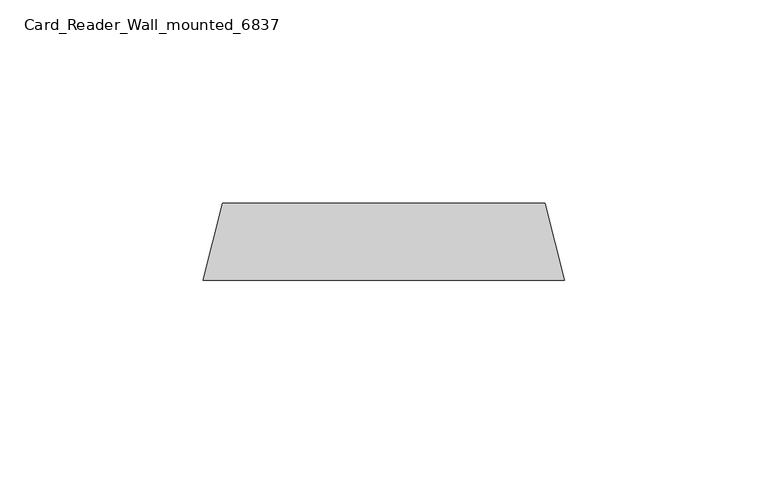
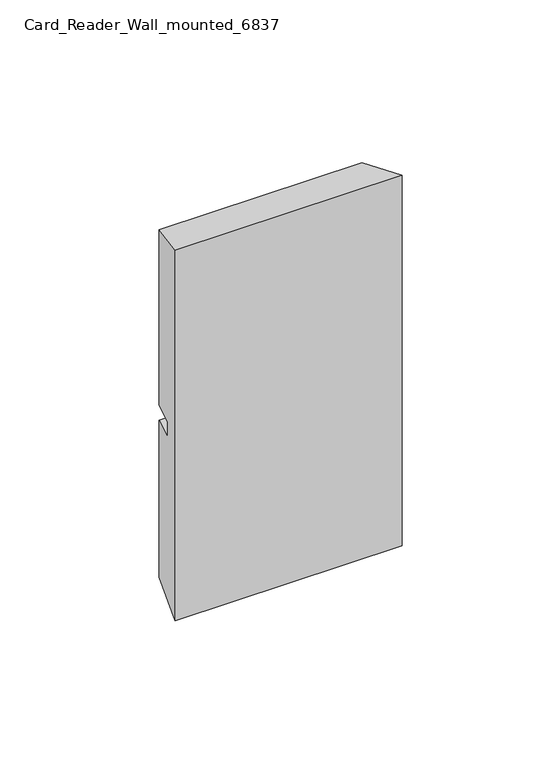
"""IFC4 building model written with IfcOpenShell, lengths in millimetres: proxy geometry, Card_Reader_Wall_mounted_6837 : swipe."""

from ifc_helpers import new_model, si_unit, origin, place, context, project, spatial, faceted_brep, source, transform, mapped, element, save


def card_reader_wall_mounted_6837_fe4ab8d8(model_context):
    return source(origin(), model_context, "Body", "Brep", [
        faceted_brep([(20.6375, 118.9392764, 1265.2375), (100.0125, 118.9392764, 1265.2375), (100.0125, 118.9392764, 1192.6911313), (20.6375, 118.9392764, 1192.6911313), (100.0125, 118.9392764, 1121.2536313), (20.6375, 118.9392764, 1121.2536313), (20.6375, 118.9392764, 1186.3411313), (100.0125, 118.9392764, 1186.3411313), (15.875, 100.0, 1270.0), (15.875, 100.0, 1116.4911313), (104.775, 100.0, 1116.4911313), (104.775, 100.0, 1270.0), (102.4977808, 109.0559335, 1186.3411313), (102.4977808, 109.0559335, 1192.6911313), (18.1522192, 109.0559335, 1192.6911313), (18.1522192, 109.0559335, 1186.3411313)], [[[0, 1, 2, 3]], [[4, 5, 6, 7]], [[8, 9, 10, 11]], [[1, 0, 8, 11]], [[11, 10, 4, 7, 12, 13, 2, 1]], [[5, 4, 10, 9]], [[9, 8, 0, 3, 14, 15, 6, 5]], [[14, 13, 12, 15]], [[15, 12, 7, 6]], [[13, 14, 3, 2]]]),
    ])


if __name__ == "__main__":
    model = new_model("IFC4")
    model_context = context("Model", 3, world=origin())
    ifc_project = project(units=[si_unit("LENGTHUNIT", "METRE", prefix="MILLI")], contexts=[model_context])
    site = spatial("IfcSite", under=ifc_project)
    building = spatial("IfcBuilding", under=site)
    placement = place(None, origin())
    card_reader_wall_mounted_6837_shape = card_reader_wall_mounted_6837_fe4ab8d8(model_context)
    element("IfcBuildingElementProxy", 1, Name="Card_Reader_Wall_mounted_6837 : swipe", ObjectType="Card_Reader_Wall_mounted_6837 : swipe", at=placement, inside=building, context=model_context, shape_type="MappedRepresentation", body=[
        mapped(card_reader_wall_mounted_6837_shape, transform((0.0, 0.0, 0.0), x_axis=(1.0, 0.0, 0.0), y_axis=(0.0, 1.0, 0.0), z_axis=(0.0, 0.0, 1.0))),
    ])
    save(model, "model.ifc")

# Revit data of these elements
# Type "Card_Reader_Wall_mounted_6837 : swipe"
#   COBie.Type.CreatedBy = "design@eagle.com"
#   COBie.Type.CreatedOn = "2016-09-13T05:47:35"
#   COBie.Type.Name = "Security Devices_Card_Reader_Wall_mounted_6837_swipe"
#   COBie.Type.Category = "23-85 30 11 : Access Controls"
#   COBie.Type.Description = ""
#   COBie.Type.Manufacturer = ""
#   COBie.Type.ModelNumber = ""
#   COBie.Type.ReplacementCost = 0
#   Width = 69.85 mm
#   Placement Height = 304.8 mm
#   Height = 114.3 mm
#   COBie.Type = yes
#   Material = Plastic - Black
#   Assembly Code = ""
# Element 1 (IfcBuildingElementProxy, "Card_Reader_Wall_mounted_6837 : swipe")
#   Materials on its faces: "Plastic - Black"
# Materials
#   "Plastic - Black": class "Plastic", colour RGB 0 0 0, transparency 0
